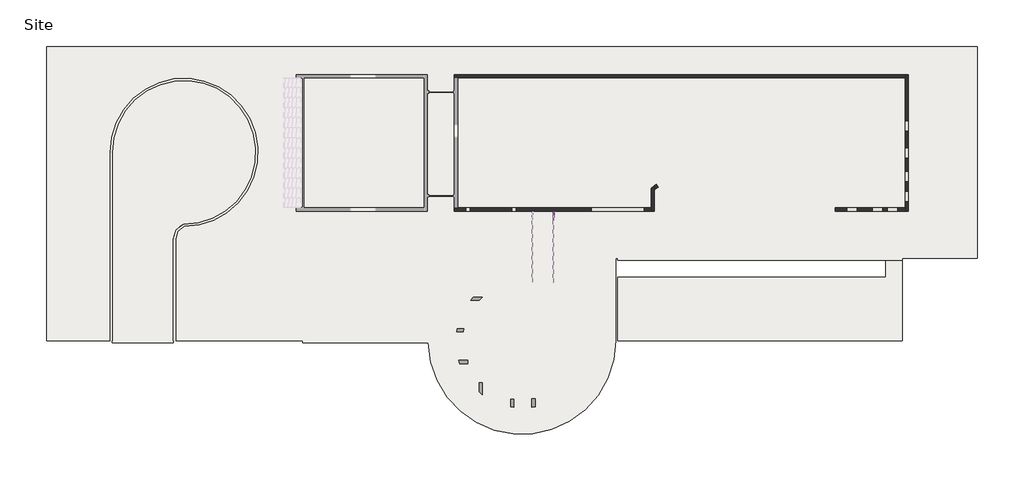
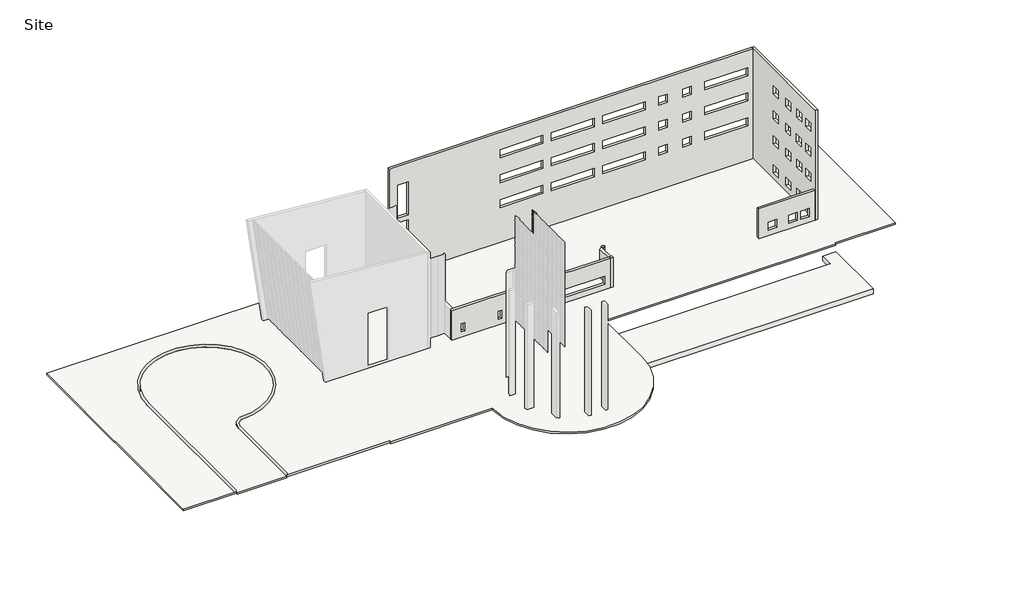
# One storey, part 4 of 4: 17 members, 6 walls, 3 slabs, 1 plate.
"""IFC4 building model written with IfcOpenShell, lengths in millimetres."""

import ifcopenshell
import ifcopenshell.guid

model = None  # the IFC model being written
_history = None  # IfcOwnerHistory: only IFC2X3 demands one
_inside = {}  # id of a spatial element -> (the spatial element, [elements in it])
_under = {}  # id of a project, library or spatial element -> (it, [spatial elements below it])
_declared = {}  # id of a project -> (the project, [libraries it declares])
_typed = {}  # id of a type object -> (the type object, [elements of that type])
_made_of = {}  # id of a material, layer set ... -> (it, [elements and type objects made of it])


def new_model(schema):
    """Start an empty IFC model of exactly this schema.

    Asked for "IFC4X3", IfcOpenShell would pick the latest addendum, in which some entities
    have other attributes; the version numbers below select the first issue.
    IFC2X3 requires an IfcOwnerHistory on every rooted entity: one is made here for all.
    """
    global model, _history
    if schema == "IFC4X3":
        model = ifcopenshell.file(schema_version=(4, 3, 0, 0))
    else:
        model = ifcopenshell.file(schema=schema)
    _inside.clear()
    _under.clear()
    _declared.clear()
    _typed.clear()
    _made_of.clear()
    _history = None
    if model.schema == "IFC2X3":
        org = make("IfcOrganization", Name="unknown")
        user = make(
            "IfcPersonAndOrganization",
            ThePerson=make("IfcPerson", FamilyName="unknown"),
            TheOrganization=org,
        )
        app = make(
            "IfcApplication",
            ApplicationDeveloper=org,
            Version="unknown",
            ApplicationFullName="unknown",
            ApplicationIdentifier="unknown",
        )
        _history = make(
            "IfcOwnerHistory",
            OwningUser=user,
            OwningApplication=app,
            ChangeAction="ADDED",
            CreationDate=0,
        )
    return model


def make(cls, **values):
    """One entity of the class cls with the attributes given. An attribute that is None is left unset."""
    return model.create_entity(
        cls, **{name: value for name, value in values.items() if value is not None}
    )


def rooted(cls, **values):
    """An entity with a GlobalId (a new one), such as an element, a storey or a relation."""
    return make(cls, GlobalId=ifcopenshell.guid.new(), OwnerHistory=_history, **values)


def si_unit(unit_type, name, prefix=None):
    """IfcSIUnit, for example si_unit("LENGTHUNIT", "METRE", prefix="MILLI")."""
    return make("IfcSIUnit", UnitType=unit_type, Prefix=prefix, Name=name)


def assignment(units):
    """IfcUnitAssignment: the units of a project."""
    return None if units is None else make("IfcUnitAssignment", Units=units)


def point(xyz):
    """IfcCartesianPoint."""
    return None if xyz is None else make("IfcCartesianPoint", Coordinates=xyz)


def direction(xyz):
    """IfcDirection."""
    return None if xyz is None else make("IfcDirection", DirectionRatios=xyz)


def frame(location, z_axis=None, x_axis=None):
    """IfcAxis2Placement3D, a coordinate frame: its origin and axes. An axis left out is left unset."""
    return make(
        "IfcAxis2Placement3D",
        Location=point(location),
        Axis=direction(z_axis),
        RefDirection=direction(x_axis),
    )


def frame_2d(location, x_axis=None):
    """IfcAxis2Placement2D, a coordinate frame in the plane: its origin and x axis."""
    return make(
        "IfcAxis2Placement2D", Location=point(location), RefDirection=direction(x_axis)
    )


def origin():
    """The frame at (0, 0, 0) with its axes left unset."""
    return frame((0.0, 0.0, 0.0))


def origin_with_axes():
    """The frame at (0, 0, 0) with the z axis (0, 0, 1) and the x axis (1, 0, 0) written out."""
    return frame((0.0, 0.0, 0.0), z_axis=(0.0, 0.0, 1.0), x_axis=(1.0, 0.0, 0.0))


def place(relative_to, where):
    """IfcLocalPlacement: puts the frame where relative to a parent placement (None: the world)."""
    return make(
        "IfcLocalPlacement", PlacementRelTo=relative_to, RelativePlacement=where
    )


def context(
    kind, dimensions, precision=None, world=None, true_north=None, identifier=None
):
    """IfcGeometricRepresentationContext, for example the 3D "Model" context."""
    return make(
        "IfcGeometricRepresentationContext",
        ContextIdentifier=identifier,
        ContextType=kind,
        CoordinateSpaceDimension=dimensions,
        Precision=precision,
        WorldCoordinateSystem=world,
        TrueNorth=true_north,
    )


def project(units=None, contexts=None):
    """IfcProject with its units and contexts."""
    return rooted(
        "IfcProject",
        Name="project",
        RepresentationContexts=contexts,
        UnitsInContext=assignment(units),
    )


def spatial(cls, under=None, at=None, **own):
    """A site, building, storey or space (cls), placed at a placement, below another one or the project."""
    s = rooted(cls, ObjectPlacement=at, **own)
    if under is not None:
        _under.setdefault(under.id(), (under, []))[1].append(s)
    return s


def polyline(points):
    """IfcPolyline through the points."""
    return make("IfcPolyline", Points=[point(p) for p in points])


def circle_curve(where, radius):
    """IfcCircle in the frame where."""
    return make("IfcCircle", Position=where, Radius=radius)


def trimmed(basis, trim1, trim2, sense, master):
    """IfcTrimmedCurve: the piece of a basis curve between two trims."""
    return make(
        "IfcTrimmedCurve",
        BasisCurve=basis,
        Trim1=trim1,
        Trim2=trim2,
        SenseAgreement=sense,
        MasterRepresentation=master,
    )


def segment(curve, same_sense, transition):
    """IfcCompositeCurveSegment."""
    return make(
        "IfcCompositeCurveSegment",
        Transition=transition,
        SameSense=same_sense,
        ParentCurve=curve,
    )


def composite_curve(segments, self_intersect=None):
    """IfcCompositeCurve: segments joined end to end."""
    return make("IfcCompositeCurve", Segments=segments, SelfIntersect=self_intersect)


def outline(outer, holes=None, kind="AREA"):
    """IfcArbitraryClosedProfileDef: a profile drawn as a closed curve; with holes, ...WithVoids."""
    if holes is None:
        return make("IfcArbitraryClosedProfileDef", ProfileType=kind, OuterCurve=outer)
    return make(
        "IfcArbitraryProfileDefWithVoids",
        ProfileType=kind,
        OuterCurve=outer,
        InnerCurves=holes,
    )


def extrude(swept, where, along, depth):
    """IfcExtrudedAreaSolid: the profile swept, set in the frame where, extruded along a direction by depth."""
    return make(
        "IfcExtrudedAreaSolid",
        SweptArea=swept,
        Position=where,
        ExtrudedDirection=direction(along),
        Depth=depth,
    )


def faces_of(points, faces, orient=None, outer=None):
    """IfcFace entities. A face is a list of loops; a loop is a list of indices into points, from 0.

    orient and outer hold one flag for each loop. By default every Orientation is true, the
    first loop of a face is its IfcFaceOuterBound and the others are IfcFaceBound.
    """
    made = []
    for i, loops in enumerate(faces):
        bounds = []
        for j, loop in enumerate(loops):
            is_outer = j == 0 if outer is None else outer[i][j]
            bounds.append(
                make(
                    "IfcFaceOuterBound" if is_outer else "IfcFaceBound",
                    Bound=make("IfcPolyLoop", Polygon=[points[k] for k in loop]),
                    Orientation=True if orient is None else orient[i][j],
                )
            )
        made.append(make("IfcFace", Bounds=bounds))
    return made


def faceted_brep(points, faces, orient=None, outer=None, voids=None):
    """IfcFacetedBrep: a solid bounded by flat faces; with voids (closed shells), ...WithVoids."""
    shared = [point(p) for p in points]
    hull = make("IfcClosedShell", CfsFaces=faces_of(shared, faces, orient, outer))
    if voids is None:
        return make("IfcFacetedBrep", Outer=hull)
    return make(
        "IfcFacetedBrepWithVoids",
        Outer=hull,
        Voids=[
            make(cls, CfsFaces=faces_of(shared, fs, o, b)) for cls, fs, o, b in voids
        ],
    )


def shape(context_of_items, identifier, shape_type, items):
    """IfcShapeRepresentation: the items that make up one representation, for example the "Body"."""
    return make(
        "IfcShapeRepresentation",
        ContextOfItems=context_of_items,
        RepresentationIdentifier=identifier,
        RepresentationType=shape_type,
        Items=items,
    )


def source(mapping_origin, context_of_items, identifier, shape_type, items):
    """IfcRepresentationMap: a shape defined once, which mapped items show again and again."""
    return make(
        "IfcRepresentationMap",
        MappingOrigin=mapping_origin,
        MappedRepresentation=shape(context_of_items, identifier, shape_type, items),
    )


def transform(
    local_origin,
    x_axis=None,
    y_axis=None,
    z_axis=None,
    scale=None,
    scale2=None,
    scale3=None,
    uniform=True,
):
    """IfcCartesianTransformationOperator3D, or its non-uniform kind. x_axis, y_axis, z_axis: its Axis1, 2, 3."""
    if uniform:
        return make(
            "IfcCartesianTransformationOperator3D",
            Axis1=direction(x_axis),
            Axis2=direction(y_axis),
            LocalOrigin=point(local_origin),
            Scale=scale,
            Axis3=direction(z_axis),
        )
    return make(
        "IfcCartesianTransformationOperator3DnonUniform",
        Axis1=direction(x_axis),
        Axis2=direction(y_axis),
        LocalOrigin=point(local_origin),
        Scale=scale,
        Axis3=direction(z_axis),
        Scale2=scale2,
        Scale3=scale3,
    )


def mapped(mapping_source, mapping_target):
    """IfcMappedItem: shows the shape of a source again, moved by a transform."""
    return make(
        "IfcMappedItem", MappingSource=mapping_source, MappingTarget=mapping_target
    )


def made_of(thing, what):
    """Note that an element or type object is made of a material, layer set ...; save() writes the relation."""
    if what is not None:
        _made_of.setdefault(what.id(), (what, []))[1].append(thing)
    return thing


def element(
    cls,
    number,
    at=None,
    inside=None,
    cuts=None,
    type_object=None,
    material=None,
    context=None,
    identifier="Body",
    shape_type=None,
    held_by="IfcProductDefinitionShape",
    body=None,
    shapes=None,
    **own,
):
    """One element of the class cls, such as IfcWall. Its Tag is "e" and its number.

    at: its placement. inside: the storey or other place that contains it. cuts: it is an
    opening in that element (IfcRelVoidsElement). A single representation is given by context,
    identifier, shape_type and body (its items); several are given by shapes. held_by: the class
    of the entity that holds the representations. save() writes the other relations.
    """
    e = rooted(cls, Tag="e%d" % number, ObjectPlacement=at, **own)
    if body is not None:
        shapes = [shape(context, identifier, shape_type, body)]
    if shapes is not None:
        e.Representation = make(held_by, Representations=shapes)
    if inside is not None:
        _inside.setdefault(inside.id(), (inside, []))[1].append(e)
    if cuts is not None:
        rooted(
            "IfcRelVoidsElement", RelatingBuildingElement=cuts, RelatedOpeningElement=e
        )
    if type_object is not None:
        _typed.setdefault(type_object.id(), (type_object, []))[1].append(e)
    return made_of(e, material)


def aggregate(whole, parts):
    """IfcRelAggregates: a whole, such as a stair, and the parts it consists of."""
    return rooted("IfcRelAggregates", RelatingObject=whole, RelatedObjects=parts)


def save(model, path):
    """Write the relations noted so far, then the file.

    IfcRelAggregates (storeys below a building ...), IfcRelContainedInSpatialStructure (elements
    in a storey), IfcRelDefinesByType, IfcRelAssociatesMaterial and IfcRelDeclares: one each for
    every whole, place, type object, material and project.
    """
    for whole, parts in _under.values():
        aggregate(whole, parts)
    for where, things in _inside.values():
        rooted(
            "IfcRelContainedInSpatialStructure",
            RelatedElements=things,
            RelatingStructure=where,
        )
    for kind, things in _typed.values():
        rooted("IfcRelDefinesByType", RelatedObjects=things, RelatingType=kind)
    for what, things in _made_of.values():
        rooted("IfcRelAssociatesMaterial", RelatedObjects=things, RelatingMaterial=what)
    for by, libraries in _declared.values():
        rooted("IfcRelDeclares", RelatingContext=by, RelatedDefinitions=libraries)
    model.write(path)


def plane_surface(at):
    """IfcPlane: the flat surface through the origin of the frame at, square to its z axis."""
    return make("IfcPlane", Position=at)


def cylinder_surface(at, radius):
    """IfcCylindricalSurface: all points at the distance radius from the z axis of the frame at."""
    return make("IfcCylindricalSurface", Position=at, Radius=radius)


def revolved_surface(curve, axis_point, axis_direction):
    """IfcSurfaceOfRevolution: the curve turned about the line through axis_point along axis_direction."""
    return make(
        "IfcSurfaceOfRevolution",
        SweptCurve=make("IfcArbitraryOpenProfileDef", ProfileType="CURVE", Curve=curve),
        AxisPosition=make("IfcAxis1Placement", Location=point(axis_point), Axis=direction(axis_direction)),
    )


def advanced_brep(points, edges, surfaces, faces):
    """IfcAdvancedBrep: a solid bounded by faces that lie on surfaces and meet in shared edges.

    An edge is (start, end): straight between two places in points (the first is 0);
    or (start, end, curve); or (start, end, curve, False) where it runs against its curve.
    A face is (place in surfaces, loops), or (place, loops, False) where it looks against
    its surface's normal. A loop lists edges by number (the first is 1), with a minus sign
    where the edge is run from its end to its start. The first loop is the outer one.
    """
    corners = [point(p) for p in points]
    vertices = [make("IfcVertexPoint", VertexGeometry=c) for c in corners]
    made = []
    for start, end, *more in edges:
        made.append(
            make(
                "IfcEdgeCurve",
                EdgeStart=vertices[start],
                EdgeEnd=vertices[end],
                EdgeGeometry=more[0] if more else make("IfcPolyline", Points=[corners[start], corners[end]]),
                SameSense=more[1] if len(more) > 1 else True,
            )
        )
    hull = []
    for where, loops, *sense in faces:
        bounds = []
        for j, loop in enumerate(loops):
            ring = [make("IfcOrientedEdge", EdgeElement=made[abs(k) - 1], Orientation=k > 0) for k in loop]
            bounds.append(
                make(
                    "IfcFaceOuterBound" if j == 0 else "IfcFaceBound",
                    Bound=make("IfcEdgeLoop", EdgeList=ring),
                    Orientation=True,
                )
            )
        hull.append(make("IfcAdvancedFace", Bounds=bounds, FaceSurface=surfaces[where], SameSense=sense[0] if sense else True))
    return make("IfcAdvancedBrep", Outer=make("IfcClosedShell", CfsFaces=hull))


def member_5d07894b(model_context):
    return source(origin(), model_context, "Body", "SweptSolid", [
        extrude(outline(polyline([(31.75, 63.5), (31.75, -63.5), (-31.75, -63.5), (-31.75, 63.5), (31.75, 63.5)])), frame((0.0, 0.0, -4629.15), z_axis=(0.0, 0.0, 1.0), x_axis=(1.0, 0.0, 0.0)), (0.0, 0.0, 1.0), 4629.15),
    ])


def member_3ba9e939(model_context):
    return source(origin(), model_context, "Body", "SweptSolid", [
        extrude(outline(polyline([(31.75, 63.5), (31.75, -63.5), (-31.75, -63.5), (-31.75, 63.5), (31.75, 63.5)])), frame((0.0, 0.0, -3746.5), z_axis=(0.0, 0.0, 1.0), x_axis=(1.0, 0.0, 0.0)), (0.0, 0.0, 1.0), 3746.5),
    ])


def member_ad567e07(model_context):
    return source(origin(), model_context, "Body", "SweptSolid", [
        extrude(outline(polyline([(31.75, 63.5), (31.75, -63.5), (-31.75, -63.5), (-31.75, 63.5), (31.75, 63.5)])), frame((0.0, 0.0, -819.15), z_axis=(0.0, 0.0, 1.0), x_axis=(1.0, 0.0, 0.0)), (0.0, 0.0, 1.0), 819.15),
    ])


def member_7db1855a(model_context):
    return source(origin(), model_context, "Body", "SweptSolid", [
        extrude(outline(polyline([(31.75, 63.5), (31.75, -63.5), (-31.75, -63.5), (-31.75, 63.5), (31.75, 63.5)])), frame((0.0, 0.0, -850.9), z_axis=(0.0, 0.0, 1.0), x_axis=(1.0, 0.0, 0.0)), (0.0, 0.0, 1.0), 850.9),
    ])


def member_ffd4c858(model_context):
    return source(origin(), model_context, "Body", "SweptSolid", [
        extrude(outline(polyline([(31.75, 63.5), (31.75, -63.5), (-31.75, -63.5), (-31.75, 63.5), (31.75, 63.5)])), frame((0.0, 0.0, -457.2), z_axis=(0.0, 0.0, 1.0), x_axis=(1.0, 0.0, 0.0)), (0.0, 0.0, 1.0), 457.2),
    ])


def member_15823cb3(model_context):
    return source(origin(), model_context, "Body", "SweptSolid", [
        extrude(outline(polyline([(0.0, 63.5), (0.0, -63.5), (-63.5, -63.5), (-63.5, 63.5), (0.0, 63.5)])), frame((0.0, 0.0, -457.2), z_axis=(0.0, 0.0, 1.0), x_axis=(1.0, 0.0, 0.0)), (0.0, 0.0, 1.0), 457.2),
    ])


def member_e9605c56(model_context):
    return source(origin(), model_context, "Body", "SweptSolid", [
        extrude(outline(polyline([(0.0, 63.5), (0.0, -63.5), (-63.5, -63.5), (-63.5, 63.5), (0.0, 63.5)])), frame((0.0, 0.0, -825.5), z_axis=(0.0, 0.0, 1.0), x_axis=(1.0, 0.0, 0.0)), (0.0, 0.0, 1.0), 825.5),
    ])


def system_panel_glazed_cc98a0ec(model_context):
    return source(origin(), model_context, "Body", "SweptSolid", [
        extrude(outline(polyline([(180.975, 19.05), (-180.975, 19.05), (-180.975, 44.45), (180.975, 44.45), (180.975, 19.05)])), origin_with_axes(), (0.0, 0.0, 1.0), 819.15),
    ])


model = new_model("IFC4")

# Units and contexts
model_context = context("Model", 3, world=origin())
ifc_project = project(units=[si_unit("LENGTHUNIT", "METRE", prefix="MILLI")], contexts=[model_context])

# Site, building, storey
site = spatial("IfcSite", under=ifc_project)
building = spatial("IfcBuilding", under=site)
storey = spatial("IfcBuildingStorey", under=building, Name="Site", Elevation=-152.4)

# Members
placement = place(None, origin())
member_shape = member_5d07894b(model_context)
element("IfcMember", 1, ObjectType="Rectangular Mullion1 : 2.5\" x 5\" rectangular", at=placement, inside=storey, context=model_context, shape_type="MappedRepresentation", body=[
    mapped(member_shape, transform((10878.8276119, 37629.311889, -88.9), x_axis=(0.0, 1.0, 0.0), y_axis=(1.0, 0.0, 0.0), z_axis=(0.0, 0.0, -1.0))),
])
member_2_shape = member_3ba9e939(model_context)
element("IfcMember", 2, ObjectType="Rectangular Mullion1 : 2.5\" x 5\" rectangular", at=placement, inside=storey, context=model_context, shape_type="MappedRepresentation", body=[
    mapped(member_2_shape, transform((10878.8276119, 37629.311889, 5518.15), x_axis=(0.0, 1.0, 0.0), y_axis=(1.0, 0.0, 0.0), z_axis=(0.0, 0.0, -1.0))),
])
element("IfcMember", 3, ObjectType="Rectangular Mullion1 : 2.5\" x 5\" rectangular", at=placement, inside=storey, context=model_context, shape_type="MappedRepresentation", body=[
    mapped(member_2_shape, transform((10878.8276119, 37629.311889, 10242.55), x_axis=(0.0, 1.0, 0.0), y_axis=(1.0, 0.0, 0.0), z_axis=(0.0, 0.0, -1.0))),
])
element("IfcMember", 4, ObjectType="Rectangular Mullion1 : 2.5\" x 5\" rectangular", at=placement, inside=storey, context=model_context, shape_type="MappedRepresentation", body=[
    mapped(member_2_shape, transform((10878.8276119, 37629.311889, 14966.95), x_axis=(0.0, 1.0, 0.0), y_axis=(1.0, 0.0, 0.0), z_axis=(0.0, 0.0, -1.0))),
])
member_3_shape = member_ad567e07(model_context)
element("IfcMember", 5, ObjectType="Rectangular Mullion1 : 2.5\" x 5\" rectangular", at=placement, inside=storey, context=model_context, shape_type="MappedRepresentation", body=[
    mapped(member_3_shape, transform((10878.8276119, 37629.311889, 18776.95), x_axis=(0.0, 1.0, 0.0), y_axis=(1.0, 0.0, 0.0), z_axis=(0.0, 0.0, -1.0))),
])
member_4_shape = member_7db1855a(model_context)
element("IfcMember", 6, ObjectType="Rectangular Mullion1 : 2.5\" x 5\" rectangular", at=placement, inside=storey, context=model_context, shape_type="MappedRepresentation", body=[
    mapped(member_4_shape, transform((10878.8276119, 37629.311889, 14052.55), x_axis=(0.0, 1.0, 0.0), y_axis=(1.0, 0.0, 0.0), z_axis=(0.0, 0.0, -1.0))),
])
element("IfcMember", 7, ObjectType="Rectangular Mullion1 : 2.5\" x 5\" rectangular", at=placement, inside=storey, context=model_context, shape_type="MappedRepresentation", body=[
    mapped(member_4_shape, transform((10878.8276119, 37629.311889, 4603.75), x_axis=(0.0, 1.0, 0.0), y_axis=(1.0, 0.0, 0.0), z_axis=(0.0, 0.0, -1.0))),
])
element("IfcMember", 8, ObjectType="Rectangular Mullion1 : 2.5\" x 5\" rectangular", at=placement, inside=storey, context=model_context, shape_type="MappedRepresentation", body=[
    mapped(member_4_shape, transform((10878.8276119, 37629.311889, 9328.15), x_axis=(0.0, 1.0, 0.0), y_axis=(1.0, 0.0, 0.0), z_axis=(0.0, 0.0, -1.0))),
])
member_5_shape = member_ffd4c858(model_context)
element("IfcMember", 9, ObjectType="Rectangular Mullion1 : 2.5\" x 5\" rectangular", at=placement, inside=storey, context=model_context, shape_type="MappedRepresentation", body=[
    mapped(member_5_shape, transform((10878.8276119, 38086.511889, 14935.2), x_axis=(0.0, 0.0, 1.0), y_axis=(1.0, 0.0, 0.0), z_axis=(0.0, 1.0, 0.0))),
])
element("IfcMember", 10, ObjectType="Rectangular Mullion1 : 2.5\" x 5\" rectangular", at=placement, inside=storey, context=model_context, shape_type="MappedRepresentation", body=[
    mapped(member_5_shape, transform((10878.8276119, 38086.511889, 10210.8), x_axis=(0.0, 0.0, 1.0), y_axis=(1.0, 0.0, 0.0), z_axis=(0.0, 1.0, 0.0))),
])
element("IfcMember", 11, ObjectType="Rectangular Mullion1 : 2.5\" x 5\" rectangular", at=placement, inside=storey, context=model_context, shape_type="MappedRepresentation", body=[
    mapped(member_5_shape, transform((10878.8276119, 38086.511889, 5486.4), x_axis=(0.0, 0.0, 1.0), y_axis=(1.0, 0.0, 0.0), z_axis=(0.0, 1.0, 0.0))),
])
element("IfcMember", 12, ObjectType="Rectangular Mullion1 : 2.5\" x 5\" rectangular", at=placement, inside=storey, context=model_context, shape_type="MappedRepresentation", body=[
    mapped(member_5_shape, transform((10878.8276119, 38086.511889, 9296.4), x_axis=(0.0, 0.0, 1.0), y_axis=(1.0, 0.0, 0.0), z_axis=(0.0, 1.0, 0.0))),
])
element("IfcMember", 13, ObjectType="Rectangular Mullion1 : 2.5\" x 5\" rectangular", at=placement, inside=storey, context=model_context, shape_type="MappedRepresentation", body=[
    mapped(member_5_shape, transform((10878.8276119, 38086.511889, 4572.0), x_axis=(0.0, 0.0, 1.0), y_axis=(1.0, 0.0, 0.0), z_axis=(0.0, 1.0, 0.0))),
])
element("IfcMember", 14, ObjectType="Rectangular Mullion1 : 2.5\" x 5\" rectangular", at=placement, inside=storey, context=model_context, shape_type="MappedRepresentation", body=[
    mapped(member_5_shape, transform((10878.8276119, 38086.511889, 14020.8), x_axis=(0.0, 0.0, 1.0), y_axis=(1.0, 0.0, 0.0), z_axis=(0.0, 1.0, 0.0))),
])
element("IfcMember", 15, ObjectType="Rectangular Mullion1 : 2.5\" x 5\" rectangular", at=placement, inside=storey, context=model_context, shape_type="MappedRepresentation", body=[
    mapped(member_5_shape, transform((10878.8276119, 38086.511889, 18745.2), x_axis=(0.0, 0.0, 1.0), y_axis=(1.0, 0.0, 0.0), z_axis=(0.0, 1.0, 0.0))),
])
member_6_shape = member_15823cb3(model_context)
element("IfcMember", 16, ObjectType="Rectangular Mullion1 : 2.5\" x 5\" rectangular", at=placement, inside=storey, context=model_context, shape_type="MappedRepresentation", body=[
    mapped(member_6_shape, transform((10878.8276119, 37629.311889, -152.4), x_axis=(0.0, 0.0, -1.0), y_axis=(1.0, 0.0, 0.0), z_axis=(0.0, -1.0, 0.0))),
])
member_7_shape = member_e9605c56(model_context)
element("IfcMember", 17, ObjectType="Rectangular Mullion1 : 2.5\" x 5\" rectangular", at=placement, inside=storey, context=model_context, shape_type="MappedRepresentation", body=[
    mapped(member_7_shape, transform((10878.8276119, 37629.311889, 19659.6), x_axis=(0.0, 0.0, 1.0), y_axis=(1.0, 0.0, 0.0), z_axis=(0.0, 1.0, 0.0))),
])

# Plate
system_panel_glazed_shape = system_panel_glazed_cc98a0ec(model_context)
element("IfcPlate", 18, ObjectType="System Panel : Glazed", at=placement, inside=storey, context=model_context, shape_type="MappedRepresentation", body=[
    mapped(system_panel_glazed_shape, transform((10878.8276119, 37842.036889, 18776.95), x_axis=(0.0, 1.0, 0.0), y_axis=(-1.0, 0.0, 0.0), z_axis=(0.0, 0.0, 1.0))),
])

# Slabs
element("IfcSlab", 19, ObjectType="a_drive", at=placement, inside=storey, context=model_context, shape_type="SweptSolid", body=[
    extrude(outline(composite_curve([segment(trimmed(circle_curve(frame_2d((-42359.2307976, 46620.911889)), 10363.2), [point((-52722.4307976, 46620.911889))], [point((-42384.6461103, 36257.743054))], False, "CARTESIAN"), True, "CONTINUOUS"), segment(trimmed(circle_curve(frame_2d((-41679.1721267, 34169.1174245)), 2204.5522361), [point((-42384.6461103, 36257.743054))], [point((-43883.2307976, 34122.4704857))], True, "CARTESIAN"), True, "CONTINUOUS"), segment(polyline([(-43883.2307976, 34122.4704857), (-43883.2307976, 19188.911889), (-52722.4307976, 19188.911889), (-52722.4307976, 46620.911889)]), True, "CONTINUOUS")], self_intersect=False)), frame((0.0, 0.0, -457.2), z_axis=(0.0, 0.0, 1.0), x_axis=(1.0, 0.0, 0.0)), (0.0, 0.0, 1.0), 304.8),
])
element("IfcSlab", 20, ObjectType="a_site paving", at=placement, inside=storey, context=model_context, shape_type="SweptSolid", body=[
    extrude(outline(composite_curve([segment(polyline([(71940.7692024, 61860.911889), (71940.7692024, 31380.911889), (61120.3692024, 31380.911889), (61120.3692024, 31076.111889), (20124.7692024, 31076.111889), (20124.7692024, 31380.911889), (19819.9692024, 31380.911889), (19819.9692024, 19493.711889)]), True, "CONTINUOUS"), segment(trimmed(circle_curve(frame_2d((6332.9997246, 19493.711889)), 13486.9694778), [point((19819.9692024, 19493.711889))], [point((-7150.5251356, 19188.911889))], False, "CARTESIAN"), True, "CONTINUOUS"), segment(polyline([(-7150.5251356, 19188.911889), (-25290.4307976, 19188.911889), (-25290.4307976, 19493.711889), (-43883.2307976, 19493.711889), (-43883.2307976, 34122.4704857)]), True, "CONTINUOUS"), segment(trimmed(circle_curve(frame_2d((-41679.1721267, 34169.1174245)), 2204.5522361), [point((-43883.2307976, 34122.4704857))], [point((-42384.6461103, 36257.743054))], False, "CARTESIAN"), True, "CONTINUOUS"), segment(trimmed(circle_curve(frame_2d((-42359.2307976, 46620.911889)), 10363.2), [point((-42384.6461103, 36257.743054))], [point((-52722.4307976, 46620.911889))], True, "CARTESIAN"), True, "CONTINUOUS"), segment(polyline([(-52722.4307976, 46620.911889), (-52722.4307976, 19493.711889), (-62171.2307976, 19493.711889), (-62171.2307976, 61860.911889), (71940.7692024, 61860.911889)]), True, "CONTINUOUS")], self_intersect=False)), frame((0.0, 0.0, -457.2), z_axis=(0.0, 0.0, 1.0), x_axis=(1.0, 0.0, 0.0)), (0.0, 0.0, 1.0), 304.8),
])
element("IfcSlab", 21, ObjectType="water feature", at=placement, inside=storey, context=model_context, shape_type="SweptSolid", body=[
    extrude(outline(polyline([(20124.7692024, 28656.761889), (58732.7692024, 28656.761889), (58732.7692024, 31076.111889), (61120.3692024, 31076.111889), (61120.3692024, 19493.711889), (20124.7692024, 19493.711889), (20124.7692024, 28656.761889)])), frame((0.0, 0.0, -2590.8), z_axis=(0.0, 0.0, 1.0), x_axis=(1.0, 0.0, 0.0)), (0.0, 0.0, 1.0), 914.4),
])

# Walls
element("IfcWall", 22, ObjectType="Stone on CMU", at=placement, inside=storey, context=model_context, shape_type="AdvancedBrep", body=[
    advanced_brep(
    [(24926.9567024, 41466.5312272, -152.4), (24926.9567024, 38618.324389, -152.4), (24926.9567024, 38164.299389, -152.4), (24926.9567024, 38164.299389, 5486.4), (24926.9567024, 38618.324389, 5486.4), (24926.9567024, 38618.324389, 5181.6), (24926.9567024, 41466.5312272, 5181.6), (25380.9817024, 41789.4772012, -152.4), (25380.9817024, 41789.4772012, 5181.6), (25380.9817024, 38618.324389, 5181.6), (25380.9817024, 38618.324389, 5486.4), (25380.9817024, 38164.299389, 5486.4), (25380.9817024, 38164.299389, -152.4), (25380.9817024, 41234.3316602, -152.4)],
    [
        (0, 1),
        (1, 2),
        (2, 3),
        (3, 4),
        (4, 5),
        (5, 6),
        (6, 0),
        (7, 8),
        (8, 9),
        (9, 10),
        (10, 11),
        (11, 12),
        (12, 13),
        (13, 7),
        (0, 7, circle_curve(frame((38486.136956, 22884.5054507, -152.4), z_axis=(0.0, 0.0, -1.0), x_axis=(1.0, 0.0, 0.0)), 23003.1095965)),
        (12, 2),
        (3, 11),
        (10, 4),
        (9, 5),
        (8, 6, circle_curve(frame((38486.136956, 22884.5054507, 5181.6), z_axis=(0.0, 0.0, 1.0), x_axis=(1.0, 0.0, 0.0)), 23003.1095965)),
    ],
    [
        plane_surface(frame((24926.9567024, 41350.796414, -152.4), z_axis=(-1.0, 0.0, 0.0), x_axis=(0.0, -1.0, 0.0))),
        plane_surface(frame((25380.9817024, 41350.796414, -152.4), z_axis=(1.0, 0.0, 0.0), x_axis=(0.0, 1.0, 0.0))),
        plane_surface(frame((24926.9567024, 41350.796414, -152.4), z_axis=(0.0, 0.0, -1.0), x_axis=(1.0, 0.0, 0.0))),
        plane_surface(frame((24926.9567024, 38391.311889, 5486.4), z_axis=(0.0, 0.0, 1.0), x_axis=(1.0, 0.0, 0.0))),
        plane_surface(frame((24926.9567024, 38618.324389, 5486.4), z_axis=(0.0, 1.0, 0.0), x_axis=(1.0, 0.0, 0.0))),
        plane_surface(frame((24926.9567024, 38618.324389, 5181.6), z_axis=(0.0, 0.0, 1.0), x_axis=(1.0, 0.0, 0.0))),
        plane_surface(frame((24696.7692024, 38164.299389, -152.4), z_axis=(0.0, -1.0, 0.0), x_axis=(1.0, 0.0, 0.0))),
        cylinder_surface(frame((38486.136956, 22884.5054507, -152.4), z_axis=(0.0, 0.0, 1.0), x_axis=(1.0, 0.0, 0.0)), 23003.1095965),
    ],
    [
        (0, [[1, 2, 3, 4, 5, 6, 7]]),
        (1, [[8, 9, 10, 11, 12, 13, 14]]),
        (2, [[-2, -1, 15, -14, -13, 16]]),
        (3, [[-4, 17, -11, 18]]),
        (4, [[-5, -18, -10, 19]]),
        (5, [[-6, -19, -9, 20]]),
        (6, [[-3, -16, -12, -17]]),
        (7, [[-7, -20, -8, -15]]),
    ],
),
])
element("IfcWall", 23, ObjectType="Stone on CMU", at=placement, inside=storey, context=model_context, shape_type="Brep", body=[
    faceted_brep([(24926.9567024, 38618.324389, 5486.4), (6799.2942024, 38618.324389, 5486.4), (6656.4192024, 38618.324389, 5486.4), (-2965.7977165, 38618.324389, 5486.4), (-3419.8227165, 38618.324389, 5486.4), (-3419.8227165, 38164.299389, 5486.4), (24926.9567024, 38164.299389, 5486.4), (24926.9567024, 38618.324389, -152.4), (-2965.7977165, 38618.324389, -152.4), (-3419.8227165, 38618.324389, -152.4), (24926.9567024, 38618.324389, 5181.6), (4884.7692024, 38618.324389, 2438.4), (4884.7692024, 38618.324389, 914.4), (5494.3692024, 38618.324389, 914.4), (5494.3692024, 38618.324389, 2438.4), (-1750.9807976, 38618.324389, 2438.4), (-1750.9807976, 38618.324389, 914.4), (-1141.3807976, 38618.324389, 914.4), (-1141.3807976, 38618.324389, 2438.4), (16314.7692024, 38618.324389, 914.4), (23934.7692024, 38618.324389, 914.4), (23934.7692024, 38618.324389, 2438.4), (16314.7692024, 38618.324389, 2438.4), (24926.9567024, 38164.299389, -152.4), (-3419.8227165, 38164.299389, -152.4), (4884.7692024, 38164.299389, 2438.4), (5494.3692024, 38164.299389, 2438.4), (5494.3692024, 38164.299389, 914.4), (4884.7692024, 38164.299389, 914.4), (-1750.9807976, 38164.299389, 2438.4), (-1141.3807976, 38164.299389, 2438.4), (-1141.3807976, 38164.299389, 914.4), (-1750.9807976, 38164.299389, 914.4), (16314.7692024, 38164.299389, 914.4), (16314.7692024, 38164.299389, 2438.4), (23934.7692024, 38164.299389, 2438.4), (23934.7692024, 38164.299389, 914.4)], [[[0, 1, 2, 3, 4, 5, 6]], [[7, 8, 9, 4, 3, 2, 1, 0, 10], [11, 12, 13, 14], [15, 16, 17, 18], [19, 20, 21, 22]], [[23, 6, 5, 24], [25, 26, 27, 28], [29, 30, 31, 32], [33, 34, 35, 36]], [[9, 8, 7, 23, 24]], [[7, 10, 0, 6, 23]], [[4, 9, 24, 5]], [[12, 11, 25, 28]], [[13, 12, 28, 27]], [[14, 13, 27, 26]], [[11, 14, 26, 25]], [[16, 15, 29, 32]], [[17, 16, 32, 31]], [[18, 17, 31, 30]], [[15, 18, 30, 29]], [[20, 19, 33, 36]], [[21, 20, 36, 35]], [[22, 21, 35, 34]], [[19, 22, 34, 33]]]),
])
element("IfcWall", 24, ObjectType="Stone on CMU", at=placement, inside=storey, context=model_context, shape_type="Brep", body=[
    faceted_brep([(61502.9567024, 38618.324389, 5486.4), (51444.5567024, 38618.324389, 5486.4), (51444.5567024, 38164.299389, 5486.4), (61502.9567024, 38164.299389, 5486.4), (61502.9567024, 38618.324389, -152.4), (51444.5567024, 38618.324389, -152.4), (51444.5567024, 38618.324389, 0.0), (51444.5567024, 38618.324389, 5181.6), (53119.3692024, 38618.324389, 2438.4), (53119.3692024, 38618.324389, 914.4), (54643.3692024, 38618.324389, 914.4), (54643.3692024, 38618.324389, 2438.4), (56776.9692024, 38618.324389, 2438.4), (56776.9692024, 38618.324389, 914.4), (58300.9692024, 38618.324389, 914.4), (58300.9692024, 38618.324389, 2438.4), (58910.5692024, 38618.324389, 2438.4), (58910.5692024, 38618.324389, 914.4), (60434.5692024, 38618.324389, 914.4), (60434.5692024, 38618.324389, 2438.4), (61502.9567024, 38164.299389, -152.4), (51444.5567024, 38164.299389, -152.4), (53119.3692024, 38164.299389, 2438.4), (54643.3692024, 38164.299389, 2438.4), (54643.3692024, 38164.299389, 914.4), (53119.3692024, 38164.299389, 914.4), (56776.9692024, 38164.299389, 2438.4), (58300.9692024, 38164.299389, 2438.4), (58300.9692024, 38164.299389, 914.4), (56776.9692024, 38164.299389, 914.4), (58910.5692024, 38164.299389, 2438.4), (60434.5692024, 38164.299389, 2438.4), (60434.5692024, 38164.299389, 914.4), (58910.5692024, 38164.299389, 914.4)], [[[0, 1, 2, 3]], [[4, 5, 6, 7, 1, 0], [8, 9, 10, 11], [12, 13, 14, 15], [16, 17, 18, 19]], [[20, 3, 2, 21], [22, 23, 24, 25], [26, 27, 28, 29], [30, 31, 32, 33]], [[5, 4, 20, 21]], [[1, 7, 6, 5, 21, 2]], [[9, 8, 22, 25]], [[10, 9, 25, 24]], [[11, 10, 24, 23]], [[8, 11, 23, 22]], [[13, 12, 26, 29]], [[14, 13, 29, 28]], [[15, 14, 28, 27]], [[12, 15, 27, 26]], [[17, 16, 30, 33]], [[18, 17, 33, 32]], [[19, 18, 32, 31]], [[16, 19, 31, 30]], [[4, 0, 3, 20]]]),
])
element("IfcWall", 25, ObjectType="Stone on CMU", at=placement, inside=storey, context=model_context, shape_type="Brep", body=[
    faceted_brep([(-3419.8227165, 57366.699389, -152.4), (-2965.7977165, 57366.699389, -152.4), (61502.9567024, 57366.699389, -152.4), (61502.9567024, 57366.699389, 20574.0), (-2965.7977165, 57366.699389, 20574.0), (-3419.8227165, 57366.699389, 20574.0), (-3419.8227165, 57366.699389, 5486.4), (-1998.6307976, 57366.699389, 10820.4), (-1998.6307976, 57366.699389, 17068.8), (-169.8307976, 57366.699389, 17068.8), (-169.8307976, 57366.699389, 10820.4), (-1998.6307976, 57366.699389, 3657.6), (-1998.6307976, 57366.699389, 9906.0), (-169.8307976, 57366.699389, 9906.0), (-169.8307976, 57366.699389, 3657.6), (42222.7692024, 57366.699389, 6400.8), (34602.7692024, 57366.699389, 6400.8), (34602.7692024, 57366.699389, 7924.8), (42222.7692024, 57366.699389, 7924.8), (42222.7692024, 57366.699389, 11125.2), (34602.7692024, 57366.699389, 11125.2), (34602.7692024, 57366.699389, 12649.2), (42222.7692024, 57366.699389, 12649.2), (42222.7692024, 57366.699389, 15849.6), (34602.7692024, 57366.699389, 15849.6), (34602.7692024, 57366.699389, 17373.6), (42222.7692024, 57366.699389, 17373.6), (33078.7692024, 57366.699389, 6400.8), (25458.7692024, 57366.699389, 6400.8), (25458.7692024, 57366.699389, 7924.8), (33078.7692024, 57366.699389, 7924.8), (33078.7692024, 57366.699389, 11125.2), (25458.7692024, 57366.699389, 11125.2), (25458.7692024, 57366.699389, 12649.2), (33078.7692024, 57366.699389, 12649.2), (33078.7692024, 57366.699389, 15849.6), (25458.7692024, 57366.699389, 15849.6), (25458.7692024, 57366.699389, 17373.6), (33078.7692024, 57366.699389, 17373.6), (23934.7692024, 57366.699389, 6400.8), (16314.7692024, 57366.699389, 6400.8), (16314.7692024, 57366.699389, 7924.8), (23934.7692024, 57366.699389, 7924.8), (23934.7692024, 57366.699389, 11125.2), (16314.7692024, 57366.699389, 11125.2), (16314.7692024, 57366.699389, 12649.2), (23934.7692024, 57366.699389, 12649.2), (23934.7692024, 57366.699389, 15849.6), (16314.7692024, 57366.699389, 15849.6), (16314.7692024, 57366.699389, 17373.6), (23934.7692024, 57366.699389, 17373.6), (60510.7692024, 57366.699389, 6400.8), (52890.7692024, 57366.699389, 6400.8), (52890.7692024, 57366.699389, 7924.8), (60510.7692024, 57366.699389, 7924.8), (60510.7692024, 57366.699389, 11125.2), (52890.7692024, 57366.699389, 11125.2), (52890.7692024, 57366.699389, 12649.2), (60510.7692024, 57366.699389, 12649.2), (60510.7692024, 57366.699389, 15849.6), (52890.7692024, 57366.699389, 15849.6), (52890.7692024, 57366.699389, 17373.6), (60510.7692024, 57366.699389, 17373.6), (50452.3692024, 57366.699389, 17373.6), (50452.3692024, 57366.699389, 15849.6), (48928.3692024, 57366.699389, 15849.6), (48928.3692024, 57366.699389, 17373.6), (46185.1692024, 57366.699389, 17373.6), (46185.1692024, 57366.699389, 15849.6), (44661.1692024, 57366.699389, 15849.6), (44661.1692024, 57366.699389, 17373.6), (50452.3692024, 57366.699389, 12649.2), (50452.3692024, 57366.699389, 11125.2), (48928.3692024, 57366.699389, 11125.2), (48928.3692024, 57366.699389, 12649.2), (46185.1692024, 57366.699389, 12649.2), (46185.1692024, 57366.699389, 11125.2), (44661.1692024, 57366.699389, 11125.2), (44661.1692024, 57366.699389, 12649.2), (50452.3692024, 57366.699389, 7924.8), (50452.3692024, 57366.699389, 6400.8), (48928.3692024, 57366.699389, 6400.8), (48928.3692024, 57366.699389, 7924.8), (46185.1692024, 57366.699389, 7924.8), (46185.1692024, 57366.699389, 6400.8), (44661.1692024, 57366.699389, 6400.8), (44661.1692024, 57366.699389, 7924.8), (61502.9567024, 57820.724389, -152.4), (-3419.8227165, 57820.724389, -152.4), (-3419.8227165, 57820.724389, 20574.0), (61502.9567024, 57820.724389, 20574.0), (-1998.6307976, 57820.724389, 17068.8), (-1998.6307976, 57820.724389, 10820.4), (-169.8307976, 57820.724389, 10820.4), (-169.8307976, 57820.724389, 17068.8), (-1998.6307976, 57820.724389, 9906.0), (-1998.6307976, 57820.724389, 3657.6), (-169.8307976, 57820.724389, 3657.6), (-169.8307976, 57820.724389, 9906.0), (42222.7692024, 57820.724389, 6400.8), (42222.7692024, 57820.724389, 7924.8), (34602.7692024, 57820.724389, 7924.8), (34602.7692024, 57820.724389, 6400.8), (42222.7692024, 57820.724389, 11125.2), (42222.7692024, 57820.724389, 12649.2), (34602.7692024, 57820.724389, 12649.2), (34602.7692024, 57820.724389, 11125.2), (42222.7692024, 57820.724389, 15849.6), (42222.7692024, 57820.724389, 17373.6), (34602.7692024, 57820.724389, 17373.6), (34602.7692024, 57820.724389, 15849.6), (33078.7692024, 57820.724389, 6400.8), (33078.7692024, 57820.724389, 7924.8), (25458.7692024, 57820.724389, 7924.8), (25458.7692024, 57820.724389, 6400.8), (33078.7692024, 57820.724389, 11125.2), (33078.7692024, 57820.724389, 12649.2), (25458.7692024, 57820.724389, 12649.2), (25458.7692024, 57820.724389, 11125.2), (33078.7692024, 57820.724389, 15849.6), (33078.7692024, 57820.724389, 17373.6), (25458.7692024, 57820.724389, 17373.6), (25458.7692024, 57820.724389, 15849.6), (23934.7692024, 57820.724389, 6400.8), (23934.7692024, 57820.724389, 7924.8), (16314.7692024, 57820.724389, 7924.8), (16314.7692024, 57820.724389, 6400.8), (23934.7692024, 57820.724389, 11125.2), (23934.7692024, 57820.724389, 12649.2), (16314.7692024, 57820.724389, 12649.2), (16314.7692024, 57820.724389, 11125.2), (23934.7692024, 57820.724389, 15849.6), (23934.7692024, 57820.724389, 17373.6), (16314.7692024, 57820.724389, 17373.6), (16314.7692024, 57820.724389, 15849.6), (60510.7692024, 57820.724389, 6400.8), (60510.7692024, 57820.724389, 7924.8), (52890.7692024, 57820.724389, 7924.8), (52890.7692024, 57820.724389, 6400.8), (60510.7692024, 57820.724389, 11125.2), (60510.7692024, 57820.724389, 12649.2), (52890.7692024, 57820.724389, 12649.2), (52890.7692024, 57820.724389, 11125.2), (60510.7692024, 57820.724389, 15849.6), (60510.7692024, 57820.724389, 17373.6), (52890.7692024, 57820.724389, 17373.6), (52890.7692024, 57820.724389, 15849.6), (50452.3692024, 57820.724389, 17373.6), (48928.3692024, 57820.724389, 17373.6), (48928.3692024, 57820.724389, 15849.6), (50452.3692024, 57820.724389, 15849.6), (46185.1692024, 57820.724389, 17373.6), (44661.1692024, 57820.724389, 17373.6), (44661.1692024, 57820.724389, 15849.6), (46185.1692024, 57820.724389, 15849.6), (50452.3692024, 57820.724389, 12649.2), (48928.3692024, 57820.724389, 12649.2), (48928.3692024, 57820.724389, 11125.2), (50452.3692024, 57820.724389, 11125.2), (46185.1692024, 57820.724389, 12649.2), (44661.1692024, 57820.724389, 12649.2), (44661.1692024, 57820.724389, 11125.2), (46185.1692024, 57820.724389, 11125.2), (50452.3692024, 57820.724389, 7924.8), (48928.3692024, 57820.724389, 7924.8), (48928.3692024, 57820.724389, 6400.8), (50452.3692024, 57820.724389, 6400.8), (46185.1692024, 57820.724389, 7924.8), (44661.1692024, 57820.724389, 7924.8), (44661.1692024, 57820.724389, 6400.8), (46185.1692024, 57820.724389, 6400.8)], [[[0, 1, 2, 3, 4, 5, 6], [7, 8, 9, 10], [11, 12, 13, 14], [15, 16, 17, 18], [19, 20, 21, 22], [23, 24, 25, 26], [27, 28, 29, 30], [31, 32, 33, 34], [35, 36, 37, 38], [39, 40, 41, 42], [43, 44, 45, 46], [47, 48, 49, 50], [51, 52, 53, 54], [55, 56, 57, 58], [59, 60, 61, 62], [63, 64, 65, 66], [67, 68, 69, 70], [71, 72, 73, 74], [75, 76, 77, 78], [79, 80, 81, 82], [83, 84, 85, 86]], [[87, 88, 89, 90], [91, 92, 93, 94], [95, 96, 97, 98], [99, 100, 101, 102], [103, 104, 105, 106], [107, 108, 109, 110], [111, 112, 113, 114], [115, 116, 117, 118], [119, 120, 121, 122], [123, 124, 125, 126], [127, 128, 129, 130], [131, 132, 133, 134], [135, 136, 137, 138], [139, 140, 141, 142], [143, 144, 145, 146], [147, 148, 149, 150], [151, 152, 153, 154], [155, 156, 157, 158], [159, 160, 161, 162], [163, 164, 165, 166], [167, 168, 169, 170]], [[0, 6, 5, 89, 88]], [[92, 91, 8, 7]], [[93, 92, 7, 10]], [[94, 93, 10, 9]], [[91, 94, 9, 8]], [[95, 12, 11, 96]], [[96, 11, 14, 97]], [[97, 14, 13, 98]], [[12, 95, 98, 13]], [[15, 18, 100, 99]], [[17, 16, 102, 101]], [[16, 15, 99, 102]], [[18, 17, 101, 100]], [[19, 22, 104, 103]], [[21, 20, 106, 105]], [[20, 19, 103, 106]], [[22, 21, 105, 104]], [[23, 26, 108, 107]], [[25, 24, 110, 109]], [[24, 23, 107, 110]], [[26, 25, 109, 108]], [[27, 30, 112, 111]], [[29, 28, 114, 113]], [[28, 27, 111, 114]], [[30, 29, 113, 112]], [[31, 34, 116, 115]], [[33, 32, 118, 117]], [[32, 31, 115, 118]], [[34, 33, 117, 116]], [[35, 38, 120, 119]], [[37, 36, 122, 121]], [[36, 35, 119, 122]], [[38, 37, 121, 120]], [[39, 42, 124, 123]], [[41, 40, 126, 125]], [[40, 39, 123, 126]], [[42, 41, 125, 124]], [[43, 46, 128, 127]], [[45, 44, 130, 129]], [[44, 43, 127, 130]], [[46, 45, 129, 128]], [[47, 50, 132, 131]], [[49, 48, 134, 133]], [[48, 47, 131, 134]], [[50, 49, 133, 132]], [[51, 54, 136, 135]], [[53, 52, 138, 137]], [[52, 51, 135, 138]], [[54, 53, 137, 136]], [[55, 58, 140, 139]], [[57, 56, 142, 141]], [[56, 55, 139, 142]], [[58, 57, 141, 140]], [[59, 62, 144, 143]], [[61, 60, 146, 145]], [[60, 59, 143, 146]], [[62, 61, 145, 144]], [[63, 66, 148, 147]], [[66, 65, 149, 148]], [[65, 64, 150, 149]], [[64, 63, 147, 150]], [[67, 70, 152, 151]], [[70, 69, 153, 152]], [[69, 68, 154, 153]], [[68, 67, 151, 154]], [[71, 74, 156, 155]], [[74, 73, 157, 156]], [[73, 72, 158, 157]], [[72, 71, 155, 158]], [[75, 78, 160, 159]], [[78, 77, 161, 160]], [[77, 76, 162, 161]], [[76, 75, 159, 162]], [[79, 82, 164, 163]], [[82, 81, 165, 164]], [[81, 80, 166, 165]], [[80, 79, 163, 166]], [[83, 86, 168, 167]], [[86, 85, 169, 168]], [[85, 84, 170, 169]], [[84, 83, 167, 170]], [[3, 2, 87, 90]], [[2, 1, 0, 88, 87]], [[5, 4, 3, 90, 89]]]),
])
element("IfcWall", 26, ObjectType="Stone on CMU", at=placement, inside=storey, context=model_context, shape_type="Brep", body=[
    faceted_brep([(61502.9567024, 57820.724389, 20574.0), (61502.9567024, 57366.699389, 20574.0), (61502.9567024, 38618.324389, 20574.0), (61502.9567024, 38164.299389, 20574.0), (61956.9817024, 38164.299389, 20574.0), (61956.9817024, 57820.724389, 20574.0), (61502.9567024, 57820.724389, -152.4), (61502.9567024, 57366.699389, -152.4), (61502.9567024, 38618.324389, -152.4), (61502.9567024, 38164.299389, -152.4), (61502.9567024, 38164.299389, 5486.4), (61502.9567024, 49643.511889, 2438.4), (61502.9567024, 49643.511889, 914.4), (61502.9567024, 51167.511889, 914.4), (61502.9567024, 51167.511889, 2438.4), (61502.9567024, 45782.711889, 2438.4), (61502.9567024, 45782.711889, 914.4), (61502.9567024, 47306.711889, 914.4), (61502.9567024, 47306.711889, 2438.4), (61502.9567024, 42379.111889, 2438.4), (61502.9567024, 42379.111889, 914.4), (61502.9567024, 43903.111889, 914.4), (61502.9567024, 43903.111889, 2438.4), (61502.9567024, 39483.511889, 2438.4), (61502.9567024, 39483.511889, 914.4), (61502.9567024, 41007.511889, 914.4), (61502.9567024, 41007.511889, 2438.4), (61502.9567024, 45782.711889, 17373.6), (61502.9567024, 45782.711889, 15849.6), (61502.9567024, 47306.711889, 15849.6), (61502.9567024, 47306.711889, 17373.6), (61502.9567024, 42379.111889, 17373.6), (61502.9567024, 42379.111889, 15849.6), (61502.9567024, 43903.111889, 15849.6), (61502.9567024, 43903.111889, 17373.6), (61502.9567024, 39483.511889, 17373.6), (61502.9567024, 39483.511889, 15849.6), (61502.9567024, 41007.511889, 15849.6), (61502.9567024, 41007.511889, 17373.6), (61502.9567024, 49643.511889, 17373.6), (61502.9567024, 49643.511889, 15849.6), (61502.9567024, 51167.511889, 15849.6), (61502.9567024, 51167.511889, 17373.6), (61502.9567024, 45782.711889, 7924.8), (61502.9567024, 45782.711889, 6400.8), (61502.9567024, 47306.711889, 6400.8), (61502.9567024, 47306.711889, 7924.8), (61502.9567024, 42379.111889, 7924.8), (61502.9567024, 42379.111889, 6400.8), (61502.9567024, 43903.111889, 6400.8), (61502.9567024, 43903.111889, 7924.8), (61502.9567024, 39483.511889, 7924.8), (61502.9567024, 39483.511889, 6400.8), (61502.9567024, 41007.511889, 6400.8), (61502.9567024, 41007.511889, 7924.8), (61502.9567024, 49643.511889, 7924.8), (61502.9567024, 49643.511889, 6400.8), (61502.9567024, 51167.511889, 6400.8), (61502.9567024, 51167.511889, 7924.8), (61502.9567024, 42448.961889, 12649.2), (61502.9567024, 42448.961889, 11125.2), (61502.9567024, 43972.961889, 11125.2), (61502.9567024, 43972.961889, 12649.2), (61502.9567024, 45801.761889, 12649.2), (61502.9567024, 45801.761889, 11125.2), (61502.9567024, 47325.761889, 11125.2), (61502.9567024, 47325.761889, 12649.2), (61502.9567024, 39553.361889, 12649.2), (61502.9567024, 39553.361889, 11125.2), (61502.9567024, 41077.361889, 11125.2), (61502.9567024, 41077.361889, 12649.2), (61502.9567024, 49592.711889, 12649.2), (61502.9567024, 49592.711889, 11125.2), (61502.9567024, 51116.711889, 11125.2), (61502.9567024, 51116.711889, 12649.2), (61956.9817024, 57820.724389, -152.4), (61956.9817024, 38164.299389, -152.4), (61956.9817024, 49643.511889, 2438.4), (61956.9817024, 51167.511889, 2438.4), (61956.9817024, 51167.511889, 914.4), (61956.9817024, 49643.511889, 914.4), (61956.9817024, 45782.711889, 2438.4), (61956.9817024, 47306.711889, 2438.4), (61956.9817024, 47306.711889, 914.4), (61956.9817024, 45782.711889, 914.4), (61956.9817024, 42379.111889, 2438.4), (61956.9817024, 43903.111889, 2438.4), (61956.9817024, 43903.111889, 914.4), (61956.9817024, 42379.111889, 914.4), (61956.9817024, 39483.511889, 2438.4), (61956.9817024, 41007.511889, 2438.4), (61956.9817024, 41007.511889, 914.4), (61956.9817024, 39483.511889, 914.4), (61956.9817024, 45782.711889, 17373.6), (61956.9817024, 47306.711889, 17373.6), (61956.9817024, 47306.711889, 15849.6), (61956.9817024, 45782.711889, 15849.6), (61956.9817024, 42379.111889, 17373.6), (61956.9817024, 43903.111889, 17373.6), (61956.9817024, 43903.111889, 15849.6), (61956.9817024, 42379.111889, 15849.6), (61956.9817024, 39483.511889, 17373.6), (61956.9817024, 41007.511889, 17373.6), (61956.9817024, 41007.511889, 15849.6), (61956.9817024, 39483.511889, 15849.6), (61956.9817024, 49643.511889, 17373.6), (61956.9817024, 51167.511889, 17373.6), (61956.9817024, 51167.511889, 15849.6), (61956.9817024, 49643.511889, 15849.6), (61956.9817024, 45782.711889, 7924.8), (61956.9817024, 47306.711889, 7924.8), (61956.9817024, 47306.711889, 6400.8), (61956.9817024, 45782.711889, 6400.8), (61956.9817024, 42379.111889, 7924.8), (61956.9817024, 43903.111889, 7924.8), (61956.9817024, 43903.111889, 6400.8), (61956.9817024, 42379.111889, 6400.8), (61956.9817024, 39483.511889, 7924.8), (61956.9817024, 41007.511889, 7924.8), (61956.9817024, 41007.511889, 6400.8), (61956.9817024, 39483.511889, 6400.8), (61956.9817024, 49643.511889, 7924.8), (61956.9817024, 51167.511889, 7924.8), (61956.9817024, 51167.511889, 6400.8), (61956.9817024, 49643.511889, 6400.8), (61956.9817024, 42448.961889, 12649.2), (61956.9817024, 43972.961889, 12649.2), (61956.9817024, 43972.961889, 11125.2), (61956.9817024, 42448.961889, 11125.2), (61956.9817024, 45801.761889, 12649.2), (61956.9817024, 47325.761889, 12649.2), (61956.9817024, 47325.761889, 11125.2), (61956.9817024, 45801.761889, 11125.2), (61956.9817024, 39553.361889, 12649.2), (61956.9817024, 41077.361889, 12649.2), (61956.9817024, 41077.361889, 11125.2), (61956.9817024, 39553.361889, 11125.2), (61956.9817024, 49592.711889, 12649.2), (61956.9817024, 51116.711889, 12649.2), (61956.9817024, 51116.711889, 11125.2), (61956.9817024, 49592.711889, 11125.2)], [[[0, 1, 2, 3, 4, 5]], [[6, 7, 8, 9, 10, 3, 2, 1, 0], [11, 12, 13, 14], [15, 16, 17, 18], [19, 20, 21, 22], [23, 24, 25, 26], [27, 28, 29, 30], [31, 32, 33, 34], [35, 36, 37, 38], [39, 40, 41, 42], [43, 44, 45, 46], [47, 48, 49, 50], [51, 52, 53, 54], [55, 56, 57, 58], [59, 60, 61, 62], [63, 64, 65, 66], [67, 68, 69, 70], [71, 72, 73, 74]], [[75, 5, 4, 76], [77, 78, 79, 80], [81, 82, 83, 84], [85, 86, 87, 88], [89, 90, 91, 92], [93, 94, 95, 96], [97, 98, 99, 100], [101, 102, 103, 104], [105, 106, 107, 108], [109, 110, 111, 112], [113, 114, 115, 116], [117, 118, 119, 120], [121, 122, 123, 124], [125, 126, 127, 128], [129, 130, 131, 132], [133, 134, 135, 136], [137, 138, 139, 140]], [[9, 8, 7, 6, 75, 76]], [[3, 10, 9, 76, 4]], [[6, 0, 5, 75]], [[12, 11, 77, 80]], [[13, 12, 80, 79]], [[14, 13, 79, 78]], [[11, 14, 78, 77]], [[16, 15, 81, 84]], [[17, 16, 84, 83]], [[18, 17, 83, 82]], [[15, 18, 82, 81]], [[20, 19, 85, 88]], [[21, 20, 88, 87]], [[22, 21, 87, 86]], [[19, 22, 86, 85]], [[24, 23, 89, 92]], [[25, 24, 92, 91]], [[26, 25, 91, 90]], [[23, 26, 90, 89]], [[28, 27, 93, 96]], [[29, 28, 96, 95]], [[30, 29, 95, 94]], [[27, 30, 94, 93]], [[32, 31, 97, 100]], [[33, 32, 100, 99]], [[34, 33, 99, 98]], [[31, 34, 98, 97]], [[36, 35, 101, 104]], [[37, 36, 104, 103]], [[38, 37, 103, 102]], [[35, 38, 102, 101]], [[40, 39, 105, 108]], [[41, 40, 108, 107]], [[42, 41, 107, 106]], [[39, 42, 106, 105]], [[44, 43, 109, 112]], [[45, 44, 112, 111]], [[46, 45, 111, 110]], [[43, 46, 110, 109]], [[48, 47, 113, 116]], [[49, 48, 116, 115]], [[50, 49, 115, 114]], [[47, 50, 114, 113]], [[52, 51, 117, 120]], [[53, 52, 120, 119]], [[54, 53, 119, 118]], [[51, 54, 118, 117]], [[56, 55, 121, 124]], [[57, 56, 124, 123]], [[58, 57, 123, 122]], [[55, 58, 122, 121]], [[60, 59, 125, 128]], [[61, 60, 128, 127]], [[62, 61, 127, 126]], [[59, 62, 126, 125]], [[64, 63, 129, 132]], [[65, 64, 132, 131]], [[66, 65, 131, 130]], [[63, 66, 130, 129]], [[68, 67, 133, 136]], [[69, 68, 136, 135]], [[70, 69, 135, 134]], [[67, 70, 134, 133]], [[72, 71, 137, 140]], [[73, 72, 140, 139]], [[74, 73, 139, 138]], [[71, 74, 138, 137]]]),
])
element("IfcWall", 27, ObjectType="Stone on CMU", at=placement, inside=storey, context=model_context, shape_type="AdvancedBrep", body=[
    advanced_brep(
    [(25380.9817024, 41234.3316602, 5334.0), (25929.0344501, 41613.6376462, 5334.0), (25676.1976468, 41990.7480433, 5334.0), (25380.9817024, 41789.4772012, 5334.0), (25380.9817024, 41234.3316602, -152.4), (25380.9817024, 41789.4772012, -152.4), (25676.1976468, 41990.7480433, -152.4), (25929.0344501, 41613.6376462, -152.4), (25380.9817024, 41789.4772012, 5181.6)],
    [
        (0, 1, circle_curve(frame((38486.136956, 22884.5054507, 5334.0), z_axis=(0.0, 0.0, -1.0), x_axis=(1.0, 0.0, 0.0)), 22549.0845965)),
        (1, 2),
        (2, 3, circle_curve(frame((38486.136956, 22884.5054507, 5334.0), z_axis=(0.0, 0.0, 1.0), x_axis=(1.0, 0.0, 0.0)), 23003.1095965)),
        (3, 0),
        (4, 5),
        (5, 6, circle_curve(frame((38486.136956, 22884.5054507, -152.4), z_axis=(0.0, 0.0, -1.0), x_axis=(1.0, 0.0, 0.0)), 23003.1095965)),
        (6, 7),
        (7, 4, circle_curve(frame((38486.136956, 22884.5054507, -152.4), z_axis=(0.0, 0.0, 1.0), x_axis=(1.0, 0.0, 0.0)), 22549.0845965)),
        (0, 4),
        (7, 1),
        (6, 2),
        (5, 8),
        (8, 3),
    ],
    [
        plane_surface(frame((61035.2215526, 22884.5054507, 5334.0), z_axis=(0.0, 0.0, 1.0), x_axis=(0.0, -1.0, 0.0))),
        plane_surface(frame((61035.2215526, 22884.5054507, -152.4), z_axis=(0.0, 0.0, -1.0), x_axis=(0.0, 1.0, 0.0))),
        revolved_surface(polyline([(61035.22155250001, 22884.5054507, -152.4), (61035.22155250001, 22884.5054507, 5334.0)]), (38486.136956, 22884.5054507, -152.4), (0.0, 0.0, -1.0)),
        plane_surface(frame((25929.0344501, 41613.6376462, 5334.0), z_axis=(0.8305939035048893, 0.5568785931067118, 0.0), x_axis=(0.0, 0.0, -1.0))),
        cylinder_surface(frame((38486.136956, 22884.5054507, -152.4), z_axis=(0.0, 0.0, 1.0), x_axis=(1.0, 0.0, 0.0)), 23003.1095965),
        plane_surface(frame((25380.9817024, 41350.796414, -152.4), z_axis=(-1.0, 0.0, 0.0), x_axis=(0.0, 1.0, 0.0))),
    ],
    [
        (0, [[1, 2, 3, 4]]),
        (1, [[5, 6, 7, 8]]),
        (2, [[-1, 9, -8, 10]]),
        (3, [[-2, -10, -7, 11]]),
        (4, [[-3, -11, -6, 12, 13]]),
        (5, [[-4, -13, -12, -5, -9]]),
    ],
),
])

save(model, "model.ifc")

# Revit data of these elements
# Type "Rectangular Mullion1 : 2.5\" x 5\" rectangular"
#   built-in parameter 1007304 = 0.416667 (stored number, unit not read)
#   built-in parameter 1007301 = 0.104167 (stored number, unit not read)
#   built-in parameter 1007300 = 0.104167 (stored number, unit not read)
# Type "System Panel : Glazed"
#   Construction Type Id = "GSP4R"
#   Analytic Construction = "1/8 in Pilkington single glazing"
#   Visual Light Transmittance = 0.9
#   Solar Heat Gain Coefficient = 0.86
#   Heat Transfer Coefficient (U) = 1.18115 BTU/(h·ft²·°F)
#   Define Thermal Properties by = 1
# Type "a_drive"
#   Function = 0
#   Layers, outside or top first: 1' - 0" "a_drive" (function 0)
# Type "a_site paving"
#   Function = 0
#   Layers, outside or top first: 1' - 0" "a_floor paving" (function 0)
# Type "water feature"
#   Function = 0
#   Layers, outside or top first: 3' - 0" "a_water" (function 0)
# Type "Stone on CMU"
#   Layers, outside or top first: 0' - 2" "Panel Granite 72x48" (function 4); 0' - 3" "Misc. Air Layers - Air Space" (function 3); 0' - 3" "Insulation / Thermal Barriers - Batt insulation" (function 3); 0' - 0" "Vapor / Moisture Barriers - Vapor Retarder" (function 100); 0' - 7 5/8" "Masonry - Concrete Masonry Units" (function 1); 0' - 1 5/8" "Metal - Furring" (function 2); 0' - 0 5/8" "Gypsum Wall Board" (function 5)
# Elements 1, 2, 3, 4, 5, 6, 7, 8, 9, 10, 11, 12, 13, 14, 15, 16, 17 (IfcMember, "Rectangular Mullion1 : 2.5\" x 5\" rectangular")
#   Phase Created = New Construction
#   Materials on its faces: "support-frame"
# Element 18 (IfcPlate, "System Panel : Glazed")
#   Phase Created = New Construction
#   Materials on its faces: "Glass"
# Element 19 (IfcSlab, "a_drive")
#   Height Offset From Level = 0' - 0"
#   Phase Created = New Construction
#   Materials on its faces: "a_drive"
# Element 20 (IfcSlab, "a_site paving")
#   Height Offset From Level = 0' - 0"
#   Phase Created = New Construction
#   Materials on its faces: "a_floor paving"
# Element 21 (IfcSlab, "water feature")
#   Height Offset From Level = -5' - 0"
#   Phase Created = New Construction
#   Materials on its faces: "a_water"
# Element 22 (IfcWall, "Stone on CMU")
#   Top Offset = 0' - 0"
#   Base Offset = 0' - 0"
#   wall height = 18' - 6"
#   Phase Created = New Construction
#   Base Constraint = Site
#   Top Constraint = Floor 2
#   Materials on its faces: "Default Wall", "Gypsum Wall Board", "Panel Granite 72x48"
# Elements 23, 24 (IfcWall, "Stone on CMU")
#   Top Offset = 0' - 0"
#   Base Offset = 0' - 0"
#   wall height = 18' - 6"
#   Phase Created = New Construction
#   Base Constraint = Site
#   Top Constraint = Floor 2
#   Materials on its faces: "Default Wall", "Panel Granite 72x48", "Gypsum Wall Board"
# Elements 25, 26 (IfcWall, "Stone on CMU")
#   Top Offset = 0' - 0"
#   Base Offset = 0' - 0"
#   wall height = 68' - 0"
#   Phase Created = New Construction
#   Base Constraint = Site
#   Top Constraint = Parapet
#   Materials on its faces: "Default Wall", "Panel Granite 72x48", "Gypsum Wall Board"
# Element 27 (IfcWall, "Stone on CMU")
#   Top Offset = -0' - 6"
#   Base Offset = 0' - 0"
#   Unconnected Height = 18' - 0"
#   wall height = 18' - 0"
#   Phase Created = New Construction
#   Materials on its faces: "Default Wall", "Panel Granite 72x48", "Gypsum Wall Board"
# Materials
#   "a_drive": class "Unassigned", colour RGB 0 0 0, transparency 0
#   "a_floor paving": class "Unassigned", colour RGB 203 186 173, transparency 0, Cost = 0
#   "a_water": class "Unassigned", colour RGB 87 85 170, transparency 0.15, Comments = "Rendering appearance not upgraded "
#   "Panel Granite 72x48": class "Stone", colour RGB 226 230 231, transparency 0, Cost = 0
#   "Misc. Air Layers - Air Space": class "Miscellaneous", colour RGB 255 255 255, transparency 0
#   "Insulation / Thermal Barriers - Batt insulation": class "Unassigned", colour RGB 127 127 127, transparency 0, Comments = "Rendering appearance not upgraded ", Cost = 0
#   "Vapor / Moisture Barriers - Vapor Retarder": class "Miscellaneous", colour RGB 127 127 127, transparency 0
#   "Masonry - Concrete Masonry Units": class "Concrete", colour RGB 227 227 227, transparency 0
#   "Metal - Furring": class "Metal", colour RGB 199 199 199, transparency 0
#   "Gypsum Wall Board": class "Generic", colour RGB 127 127 127, transparency 0, Description = "Gypsum Wall Board", Cost = 0
#   "support-frame": class "Unassigned", colour RGB 233 233 233, transparency 0, Cost = 0
#   "Glass": class "Glass", colour RGB 0 128 192, transparency 0.75, Description = "Soda Lime Glass", Cost = 0
#   "Default Wall": class "Miscellaneous", colour RGB 128 128 128, transparency 0, Cost = 0
